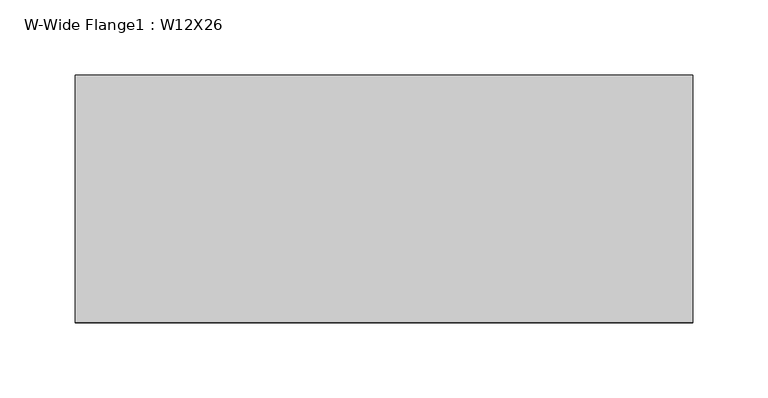
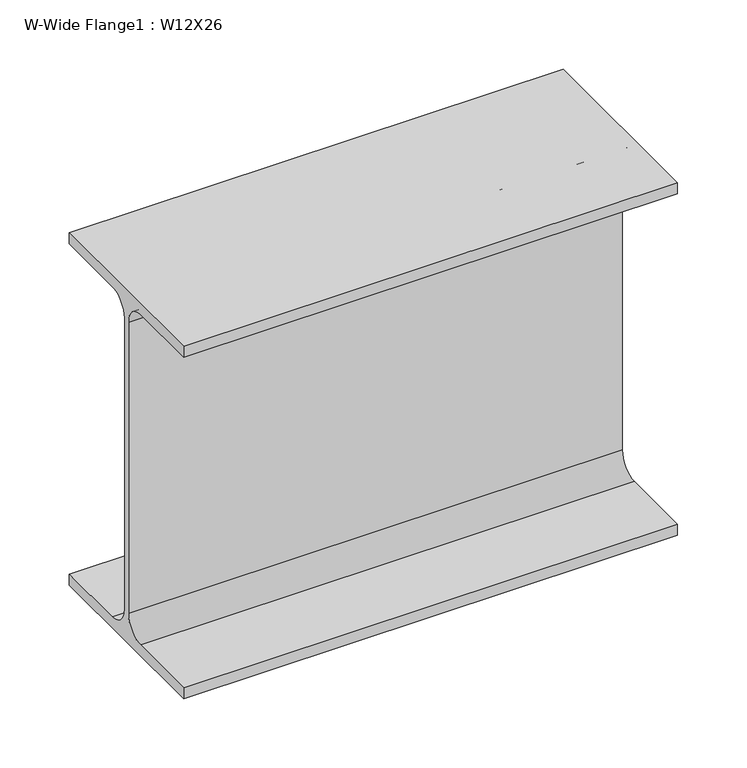
"""IFC4 building model written with IfcOpenShell, lengths in millimetres: beam geometry, W-Wide Flange1 : W12X26."""

import ifcopenshell
import ifcopenshell.guid

model = None  # the IFC model being written
_history = None  # IfcOwnerHistory: only IFC2X3 demands one
_inside = {}  # id of a spatial element -> (the spatial element, [elements in it])
_under = {}  # id of a project, library or spatial element -> (it, [spatial elements below it])
_declared = {}  # id of a project -> (the project, [libraries it declares])
_typed = {}  # id of a type object -> (the type object, [elements of that type])
_made_of = {}  # id of a material, layer set ... -> (it, [elements and type objects made of it])


def new_model(schema):
    """Start an empty IFC model of exactly this schema.

    Asked for "IFC4X3", IfcOpenShell would pick the latest addendum, in which some entities
    have other attributes; the version numbers below select the first issue.
    IFC2X3 requires an IfcOwnerHistory on every rooted entity: one is made here for all.
    """
    global model, _history
    if schema == "IFC4X3":
        model = ifcopenshell.file(schema_version=(4, 3, 0, 0))
    else:
        model = ifcopenshell.file(schema=schema)
    _inside.clear()
    _under.clear()
    _declared.clear()
    _typed.clear()
    _made_of.clear()
    _history = None
    if model.schema == "IFC2X3":
        org = make("IfcOrganization", Name="unknown")
        user = make(
            "IfcPersonAndOrganization",
            ThePerson=make("IfcPerson", FamilyName="unknown"),
            TheOrganization=org,
        )
        app = make(
            "IfcApplication",
            ApplicationDeveloper=org,
            Version="unknown",
            ApplicationFullName="unknown",
            ApplicationIdentifier="unknown",
        )
        _history = make(
            "IfcOwnerHistory",
            OwningUser=user,
            OwningApplication=app,
            ChangeAction="ADDED",
            CreationDate=0,
        )
    return model


def make(cls, **values):
    """One entity of the class cls with the attributes given. An attribute that is None is left unset."""
    return model.create_entity(
        cls, **{name: value for name, value in values.items() if value is not None}
    )


def rooted(cls, **values):
    """An entity with a GlobalId (a new one), such as an element, a storey or a relation."""
    return make(cls, GlobalId=ifcopenshell.guid.new(), OwnerHistory=_history, **values)


def si_unit(unit_type, name, prefix=None):
    """IfcSIUnit, for example si_unit("LENGTHUNIT", "METRE", prefix="MILLI")."""
    return make("IfcSIUnit", UnitType=unit_type, Prefix=prefix, Name=name)


def assignment(units):
    """IfcUnitAssignment: the units of a project."""
    return None if units is None else make("IfcUnitAssignment", Units=units)


def point(xyz):
    """IfcCartesianPoint."""
    return None if xyz is None else make("IfcCartesianPoint", Coordinates=xyz)


def direction(xyz):
    """IfcDirection."""
    return None if xyz is None else make("IfcDirection", DirectionRatios=xyz)


def frame(location, z_axis=None, x_axis=None):
    """IfcAxis2Placement3D, a coordinate frame: its origin and axes. An axis left out is left unset."""
    return make(
        "IfcAxis2Placement3D",
        Location=point(location),
        Axis=direction(z_axis),
        RefDirection=direction(x_axis),
    )


def frame_2d(location, x_axis=None):
    """IfcAxis2Placement2D, a coordinate frame in the plane: its origin and x axis."""
    return make(
        "IfcAxis2Placement2D", Location=point(location), RefDirection=direction(x_axis)
    )


def origin():
    """The frame at (0, 0, 0) with its axes left unset."""
    return frame((0.0, 0.0, 0.0))


def place(relative_to, where):
    """IfcLocalPlacement: puts the frame where relative to a parent placement (None: the world)."""
    return make(
        "IfcLocalPlacement", PlacementRelTo=relative_to, RelativePlacement=where
    )


def context(
    kind, dimensions, precision=None, world=None, true_north=None, identifier=None
):
    """IfcGeometricRepresentationContext, for example the 3D "Model" context."""
    return make(
        "IfcGeometricRepresentationContext",
        ContextIdentifier=identifier,
        ContextType=kind,
        CoordinateSpaceDimension=dimensions,
        Precision=precision,
        WorldCoordinateSystem=world,
        TrueNorth=true_north,
    )


def project(units=None, contexts=None):
    """IfcProject with its units and contexts."""
    return rooted(
        "IfcProject",
        Name="project",
        RepresentationContexts=contexts,
        UnitsInContext=assignment(units),
    )


def spatial(cls, under=None, at=None, **own):
    """A site, building, storey or space (cls), placed at a placement, below another one or the project."""
    s = rooted(cls, ObjectPlacement=at, **own)
    if under is not None:
        _under.setdefault(under.id(), (under, []))[1].append(s)
    return s


def polyline(points):
    """IfcPolyline through the points."""
    return make("IfcPolyline", Points=[point(p) for p in points])


def circle_curve(where, radius):
    """IfcCircle in the frame where."""
    return make("IfcCircle", Position=where, Radius=radius)


def trimmed(basis, trim1, trim2, sense, master):
    """IfcTrimmedCurve: the piece of a basis curve between two trims."""
    return make(
        "IfcTrimmedCurve",
        BasisCurve=basis,
        Trim1=trim1,
        Trim2=trim2,
        SenseAgreement=sense,
        MasterRepresentation=master,
    )


def segment(curve, same_sense, transition):
    """IfcCompositeCurveSegment."""
    return make(
        "IfcCompositeCurveSegment",
        Transition=transition,
        SameSense=same_sense,
        ParentCurve=curve,
    )


def composite_curve(segments, self_intersect=None):
    """IfcCompositeCurve: segments joined end to end."""
    return make("IfcCompositeCurve", Segments=segments, SelfIntersect=self_intersect)


def outline(outer, holes=None, kind="AREA"):
    """IfcArbitraryClosedProfileDef: a profile drawn as a closed curve; with holes, ...WithVoids."""
    if holes is None:
        return make("IfcArbitraryClosedProfileDef", ProfileType=kind, OuterCurve=outer)
    return make(
        "IfcArbitraryProfileDefWithVoids",
        ProfileType=kind,
        OuterCurve=outer,
        InnerCurves=holes,
    )


def extrude(swept, where, along, depth):
    """IfcExtrudedAreaSolid: the profile swept, set in the frame where, extruded along a direction by depth."""
    return make(
        "IfcExtrudedAreaSolid",
        SweptArea=swept,
        Position=where,
        ExtrudedDirection=direction(along),
        Depth=depth,
    )


def shape(context_of_items, identifier, shape_type, items):
    """IfcShapeRepresentation: the items that make up one representation, for example the "Body"."""
    return make(
        "IfcShapeRepresentation",
        ContextOfItems=context_of_items,
        RepresentationIdentifier=identifier,
        RepresentationType=shape_type,
        Items=items,
    )


def source(mapping_origin, context_of_items, identifier, shape_type, items):
    """IfcRepresentationMap: a shape defined once, which mapped items show again and again."""
    return make(
        "IfcRepresentationMap",
        MappingOrigin=mapping_origin,
        MappedRepresentation=shape(context_of_items, identifier, shape_type, items),
    )


def transform(
    local_origin,
    x_axis=None,
    y_axis=None,
    z_axis=None,
    scale=None,
    scale2=None,
    scale3=None,
    uniform=True,
):
    """IfcCartesianTransformationOperator3D, or its non-uniform kind. x_axis, y_axis, z_axis: its Axis1, 2, 3."""
    if uniform:
        return make(
            "IfcCartesianTransformationOperator3D",
            Axis1=direction(x_axis),
            Axis2=direction(y_axis),
            LocalOrigin=point(local_origin),
            Scale=scale,
            Axis3=direction(z_axis),
        )
    return make(
        "IfcCartesianTransformationOperator3DnonUniform",
        Axis1=direction(x_axis),
        Axis2=direction(y_axis),
        LocalOrigin=point(local_origin),
        Scale=scale,
        Axis3=direction(z_axis),
        Scale2=scale2,
        Scale3=scale3,
    )


def mapped(mapping_source, mapping_target):
    """IfcMappedItem: shows the shape of a source again, moved by a transform."""
    return make(
        "IfcMappedItem", MappingSource=mapping_source, MappingTarget=mapping_target
    )


def made_of(thing, what):
    """Note that an element or type object is made of a material, layer set ...; save() writes the relation."""
    if what is not None:
        _made_of.setdefault(what.id(), (what, []))[1].append(thing)
    return thing


def element(
    cls,
    number,
    at=None,
    inside=None,
    cuts=None,
    type_object=None,
    material=None,
    context=None,
    identifier="Body",
    shape_type=None,
    held_by="IfcProductDefinitionShape",
    body=None,
    shapes=None,
    **own,
):
    """One element of the class cls, such as IfcWall. Its Tag is "e" and its number.

    at: its placement. inside: the storey or other place that contains it. cuts: it is an
    opening in that element (IfcRelVoidsElement). A single representation is given by context,
    identifier, shape_type and body (its items); several are given by shapes. held_by: the class
    of the entity that holds the representations. save() writes the other relations.
    """
    e = rooted(cls, Tag="e%d" % number, ObjectPlacement=at, **own)
    if body is not None:
        shapes = [shape(context, identifier, shape_type, body)]
    if shapes is not None:
        e.Representation = make(held_by, Representations=shapes)
    if inside is not None:
        _inside.setdefault(inside.id(), (inside, []))[1].append(e)
    if cuts is not None:
        rooted(
            "IfcRelVoidsElement", RelatingBuildingElement=cuts, RelatedOpeningElement=e
        )
    if type_object is not None:
        _typed.setdefault(type_object.id(), (type_object, []))[1].append(e)
    return made_of(e, material)


def aggregate(whole, parts):
    """IfcRelAggregates: a whole, such as a stair, and the parts it consists of."""
    return rooted("IfcRelAggregates", RelatingObject=whole, RelatedObjects=parts)


def save(model, path):
    """Write the relations noted so far, then the file.

    IfcRelAggregates (storeys below a building ...), IfcRelContainedInSpatialStructure (elements
    in a storey), IfcRelDefinesByType, IfcRelAssociatesMaterial and IfcRelDeclares: one each for
    every whole, place, type object, material and project.
    """
    for whole, parts in _under.values():
        aggregate(whole, parts)
    for where, things in _inside.values():
        rooted(
            "IfcRelContainedInSpatialStructure",
            RelatedElements=things,
            RelatingStructure=where,
        )
    for kind, things in _typed.values():
        rooted("IfcRelDefinesByType", RelatedObjects=things, RelatingType=kind)
    for what, things in _made_of.values():
        rooted("IfcRelAssociatesMaterial", RelatedObjects=things, RelatingMaterial=what)
    for by, libraries in _declared.values():
        rooted("IfcRelDeclares", RelatingContext=by, RelatedDefinitions=libraries)
    model.write(path)


def w_wide_flange1_w12x26_5f533c06(model_context):
    return source(origin(), model_context, "Body", "SweptSolid", [
        extrude(outline(composite_curve([segment(polyline([(82.423, -145.288), (82.423, -154.94), (-82.423, -154.94), (-82.423, -145.288), (-20.2565, -145.288)]), True, "CONTINUOUS"), segment(trimmed(circle_curve(frame_2d((-20.2565, -127.9525)), 17.3355), [point((-20.2565, -145.288))], [point((-2.921, -127.9525))], True, "CARTESIAN"), True, "CONTINUOUS"), segment(polyline([(-2.921, -127.9525), (-2.921, 127.9525)]), True, "CONTINUOUS"), segment(trimmed(circle_curve(frame_2d((-20.2565, 127.9525)), 17.3355), [point((-2.921, 127.9525))], [point((-20.2565, 145.288))], True, "CARTESIAN"), True, "CONTINUOUS"), segment(polyline([(-20.2565, 145.288), (-82.423, 145.288), (-82.423, 154.94), (82.423, 154.94), (82.423, 145.288), (20.2565, 145.288)]), True, "CONTINUOUS"), segment(trimmed(circle_curve(frame_2d((20.2565, 127.9525)), 17.3355), [point((20.2565, 145.288))], [point((2.921, 127.9525))], True, "CARTESIAN"), True, "CONTINUOUS"), segment(polyline([(2.921, 127.9525), (2.921, -127.9525)]), True, "CONTINUOUS"), segment(trimmed(circle_curve(frame_2d((20.2565, -127.9525)), 17.3355), [point((2.921, -127.9525))], [point((20.2565, -145.288))], True, "CARTESIAN"), True, "CONTINUOUS"), segment(polyline([(20.2565, -145.288), (82.423, -145.288)]), True, "CONTINUOUS")], self_intersect=False)), frame((-193.323775, 0.0, 0.0), z_axis=(1.0, 0.0, 0.0), x_axis=(0.0, 1.0, 0.0)), (0.0, 0.0, 1.0), 410.9438375),
    ])


if __name__ == "__main__":
    model = new_model("IFC4")
    model_context = context("Model", 3, world=origin())
    ifc_project = project(units=[si_unit("LENGTHUNIT", "METRE", prefix="MILLI")], contexts=[model_context])
    site = spatial("IfcSite", under=ifc_project)
    building = spatial("IfcBuilding", under=site)
    placement = place(None, origin())
    w_wide_flange1_w12x26_shape = w_wide_flange1_w12x26_5f533c06(model_context)
    element("IfcBeam", 1, ObjectType="W-Wide Flange1 : W12X26", at=placement, inside=building, context=model_context, shape_type="MappedRepresentation", body=[
        mapped(w_wide_flange1_w12x26_shape, transform((0.0, 0.0, 0.0), x_axis=(1.0, 0.0, 0.0), y_axis=(0.0, 1.0, 0.0), z_axis=(0.0, 0.0, 1.0))),
    ])
    save(model, "model.ifc")

# Revit data of these elements
# Type "W-Wide Flange1 : W12X26"
#   Assembly Code = "B10"
#   W = 26
#   Start Extension Calculation [instance default] = 10' - 0"
#   Start Extension [instance default] = -0' - 0 1/2"
#   End Extension Calculation [instance default] = 10' - 0"
#   End Extension [instance default] = -0' - 0 1/2"
#   Length [instance default] = 5' - 0"
#   bf = 0' - 6.49"
#   d = 1' - 0.2"
#   k = 0' - 1 1/16"
#   k2 = 0' - 0.6825"
#   tf = 0' - 0.38"
#   tw = 0' - 0.23"
#   A = 0.053125 SF
#   Structural Material [instance default] = Metal - Steel - ASTM A992
# Element 1 (IfcBeam, "W-Wide Flange1 : W12X26")
#   Materials on its faces: "Metal - Steel - ASTM A992"
# Materials
#   "Metal - Steel - ASTM A992": class "Metal", colour RGB 199 199 199, transparency 0
